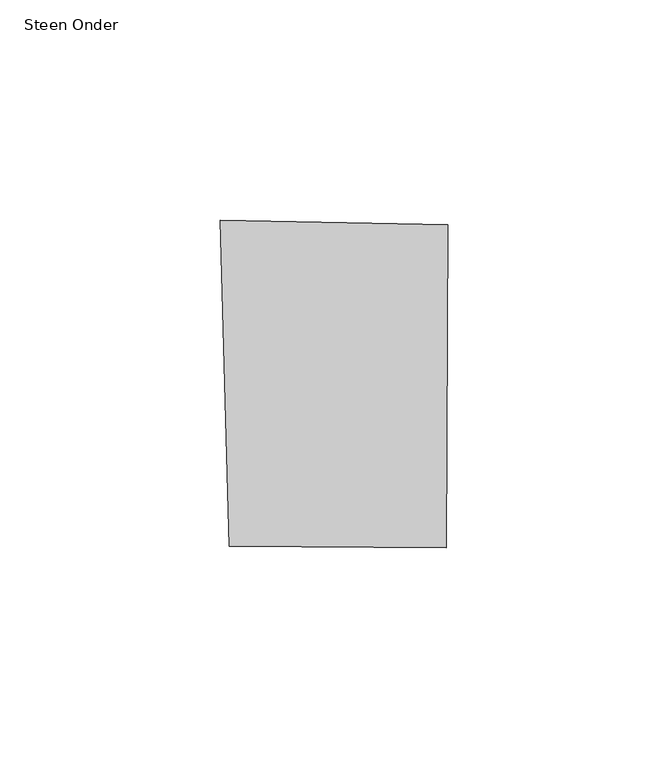
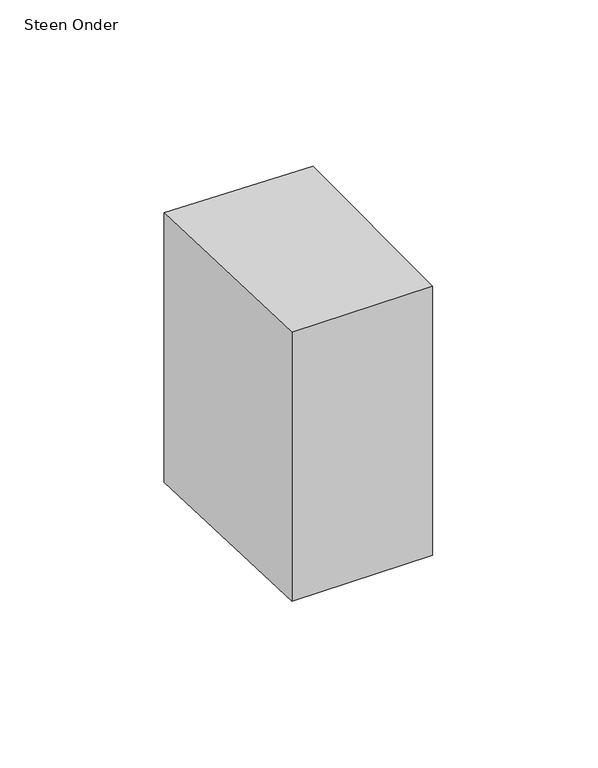
"""IFC4 building model written with IfcOpenShell, lengths in millimetres: proxy geometry, 00_GMA_steen_versie_4 : Steen Onder."""

from ifc_helpers import new_model, si_unit, origin, origin_with_axes, place, context, project, spatial, polyline, outline, extrude, source, transform, mapped, element, save


def steen_onder_60f660a6(model_context):
    return source(origin(), model_context, "Body", "SweptSolid", [
        extrude(outline(polyline([(100.690137, 103.0203232), (100.4012378, 29.5685133), (51.1085668, 29.9283717), (48.9960091, 104.0760993), (100.690137, 103.0203232)])), origin_with_axes(), (0.0, 0.0, 1.0), 100.0),
    ])


if __name__ == "__main__":
    model = new_model("IFC4")
    model_context = context("Model", 3, world=origin())
    ifc_project = project(units=[si_unit("LENGTHUNIT", "METRE", prefix="MILLI")], contexts=[model_context])
    site = spatial("IfcSite", under=ifc_project)
    building = spatial("IfcBuilding", under=site)
    placement = place(None, origin())
    steen_onder_shape = steen_onder_60f660a6(model_context)
    element("IfcBuildingElementProxy", 1, Name="00_GMA_steen_versie_4 : Steen Onder", ObjectType="00_GMA_steen_versie_4 : Steen Onder", at=placement, inside=building, context=model_context, shape_type="MappedRepresentation", body=[
        mapped(steen_onder_shape, transform((0.0, 0.0, 0.0), x_axis=(1.0, 0.0, 0.0), y_axis=(0.0, 1.0, 0.0), z_axis=(0.0, 0.0, 1.0))),
    ])
    save(model, "model.ifc")

# Revit data of these elements
# Type "00_GMA_steen_versie_4 : Steen Onder"
#   StootVoegHalfBoven [instance default] = 5 mm
#   StootVoegHalf [instance default] = 5 mm
#   StootVoegBreedteOnder = 10 mm
#   StootVoegBreedteBoven = 10 mm
#   Steendikte = 100 mm
#   LintVoegOnderHalf = 0 mm
#   LintVoegOnder = 0 mm
#   LintVoegBovenHalf = 5 mm
#   LintVoegBoven = 10 mm
#   materiaal = none
#   MateriaalVoeg = none
#   Default Elevation = 0
